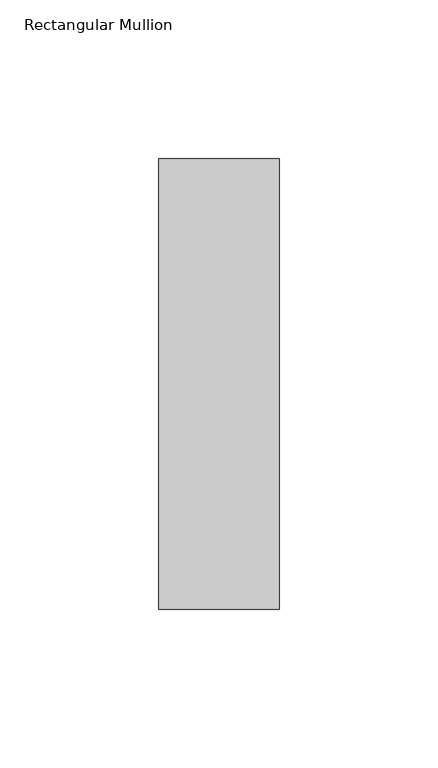
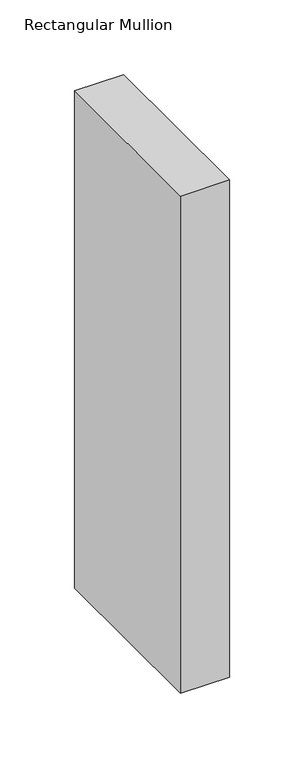
"""IFC4 building model written with IfcOpenShell, lengths in millimetres: member geometry, Rectangular Mullion : NLRS_21_CWM_hsb-regel 38x142_gen_rsf."""

from ifc_helpers import new_model, si_unit, frame, origin, place, context, project, spatial, polyline, outline, extrude, source, transform, mapped, element, save


def rectangular_mullion_2a836202(model_context):
    return source(origin(), model_context, "Body", "SweptSolid", [
        extrude(outline(polyline([(0.0, -71.0), (-38.0, -71.0), (-38.0, 71.0), (0.0, 71.0), (0.0, -71.0)])), frame((0.0, 0.0, -407.0000003), z_axis=(0.0, 0.0, 1.0), x_axis=(1.0, 0.0, 0.0)), (0.0, 0.0, 1.0), 407.0000003),
    ])


if __name__ == "__main__":
    model = new_model("IFC4")
    model_context = context("Model", 3, world=origin())
    ifc_project = project(units=[si_unit("LENGTHUNIT", "METRE", prefix="MILLI")], contexts=[model_context])
    site = spatial("IfcSite", under=ifc_project)
    building = spatial("IfcBuilding", under=site)
    placement = place(None, origin())
    rectangular_mullion_shape = rectangular_mullion_2a836202(model_context)
    element("IfcMember", 1, ObjectType="Rectangular Mullion : NLRS_21_CWM_hsb-regel 38x142_gen_rsf", at=placement, inside=building, context=model_context, shape_type="MappedRepresentation", body=[
        mapped(rectangular_mullion_shape, transform((0.0, 0.0, 0.0), x_axis=(1.0, 0.0, 0.0), y_axis=(0.0, 1.0, 0.0), z_axis=(0.0, 0.0, 1.0))),
    ])
    save(model, "model.ifc")

# Revit data of these elements
# Type "Rectangular Mullion : NLRS_21_CWM_hsb-regel 38x142_gen_rsf"
#   Export Type to IFC As = "IfcWall"
#   Type IfcGUID = "07M7mRoiH1CR8m_RSKIwpF"
#   Assembly Code = "21.10"
#   built-in parameter 1007322 = 0.465879 (stored number, unit not read)
#   built-in parameter 1007321 = 0.062336 (stored number, unit not read)
#   built-in parameter 1007320 = 0.062336 (stored number, unit not read)
# Element 1 (IfcMember, "Rectangular Mullion : NLRS_21_CWM_hsb-regel 38x142_gen_rsf")
#   Materials on its faces: "NLRS_i2_hout naaldhout vuren_gen_rsf"
# Materials
#   "NLRS_i2_hout naaldhout vuren_gen_rsf": class "I - Hout", colour RGB 234 199 147, transparency 0, Keynote = "i2", Manufacturer = "Revit Standards Foundation", URL = "www.revitstandards.org", Description = "hout vuren", Cost = 0
